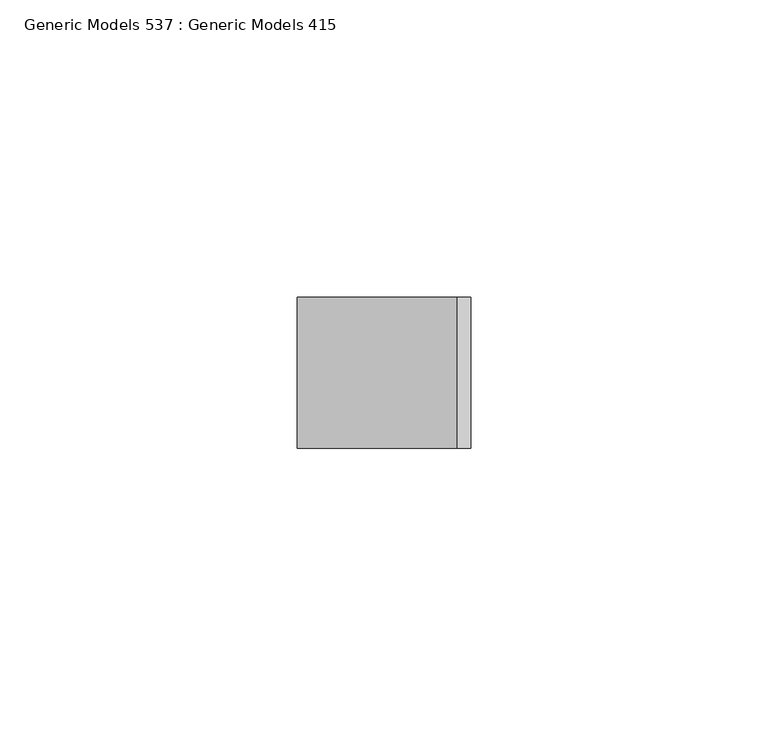
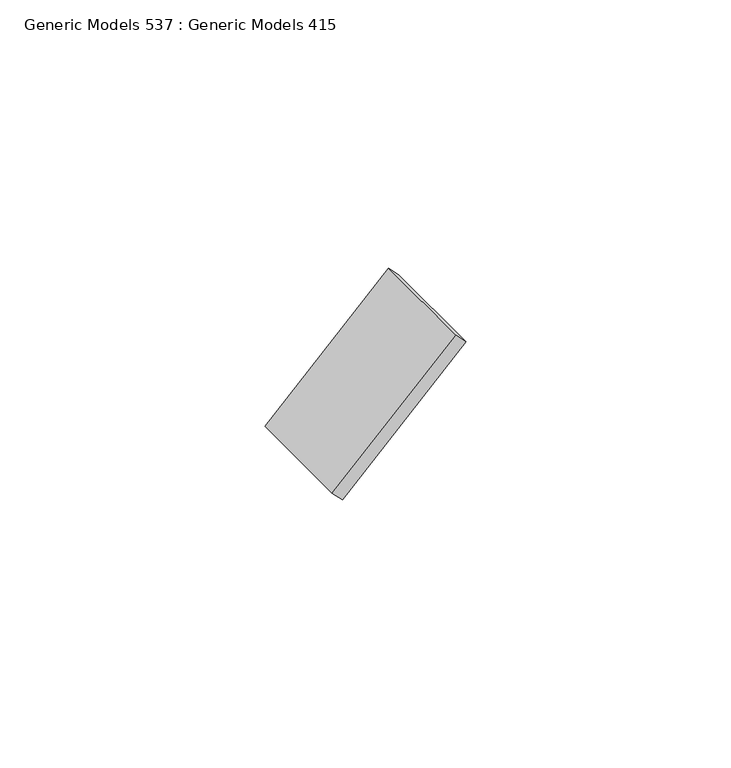
"""IFC4 building model written with IfcOpenShell, lengths in millimetres: proxy geometry, Generic Models 537 : Generic Models 415."""

from ifc_helpers import new_model, si_unit, frame, origin, place, context, project, spatial, polyline, outline, extrude, source, transform, mapped, element, save


def generic_models_537_generic_models_415_124e1c67(model_context):
    return source(origin(), model_context, "Body", "SweptSolid", [
        extrude(outline(polyline([(0.0, -3.175), (0.0, 0.0), (25.4, 0.0), (25.4, -3.175), (0.0, -3.175)])), frame((7848.0411784, 4501.3863946, 125130.8849742), z_axis=(0.7071067811867181, 0.0, 0.707106781186377), x_axis=(0.0, -1.0, 0.0)), (0.0, 0.0, 1.0), 38.1),
    ])


if __name__ == "__main__":
    model = new_model("IFC4")
    model_context = context("Model", 3, world=origin())
    ifc_project = project(units=[si_unit("LENGTHUNIT", "METRE", prefix="MILLI")], contexts=[model_context])
    site = spatial("IfcSite", under=ifc_project)
    building = spatial("IfcBuilding", under=site)
    placement = place(None, origin())
    generic_models_537_generic_models_415_shape = generic_models_537_generic_models_415_124e1c67(model_context)
    element("IfcBuildingElementProxy", 1, Name="Generic Models 537 : Generic Models 415", ObjectType="Generic Models 537 : Generic Models 415", at=placement, inside=building, context=model_context, shape_type="MappedRepresentation", body=[
        mapped(generic_models_537_generic_models_415_shape, transform((0.0, 0.0, 0.0), x_axis=(1.0, 0.0, 0.0), y_axis=(0.0, 1.0, 0.0), z_axis=(0.0, 0.0, 1.0))),
    ])
    save(model, "model.ifc")

# Revit data of these elements
# Element 1 (IfcBuildingElementProxy, "Generic Models 537 : Generic Models 415")
#   Materials on its faces: "_WELDED STEEL TABS FOR LOUVER ATTACHMENT"
# Materials
#   "_WELDED STEEL TABS FOR LOUVER ATTACHMENT": class "Metal", colour RGB 199 199 199, transparency 0, Description = "Structural steel 50ksi", Cost = 0
